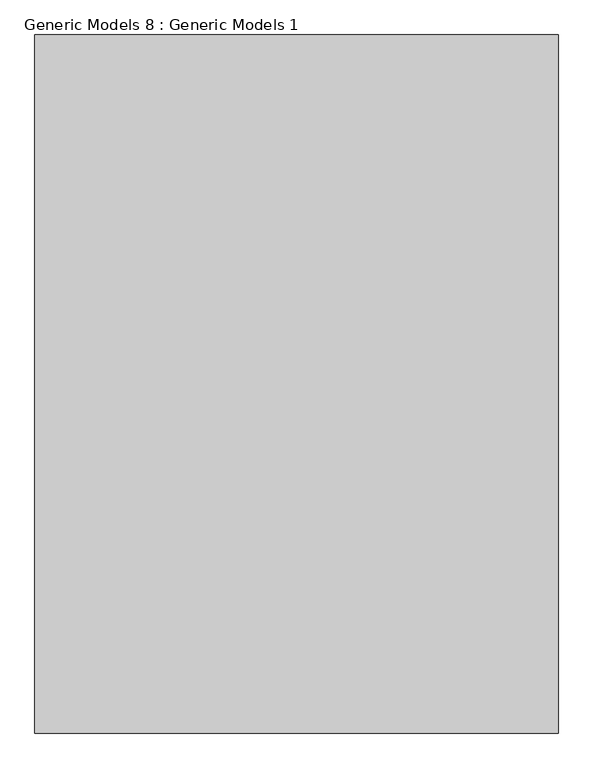
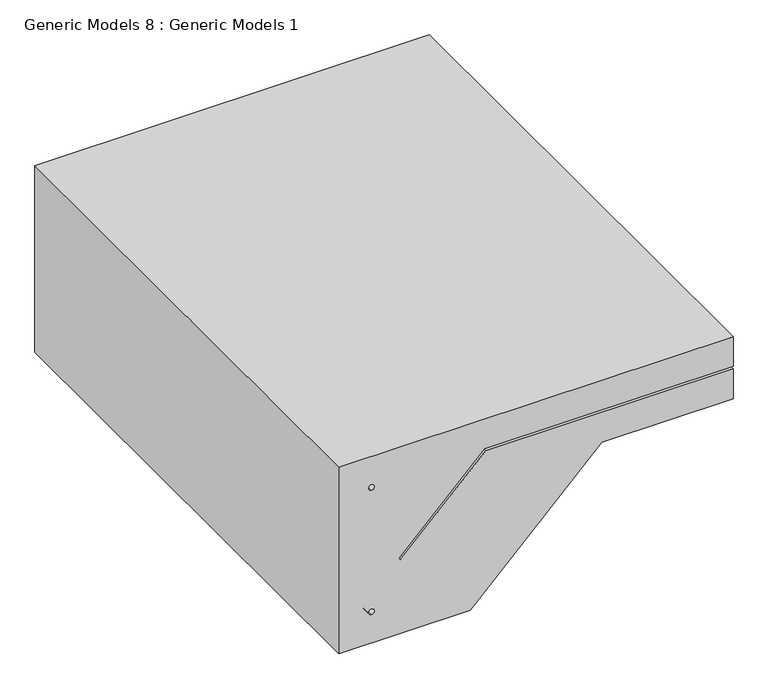
"""IFC4 building model written with IfcOpenShell, lengths in millimetres: proxy geometry, Generic Models 8 : Generic Models 1."""

import ifcopenshell
import ifcopenshell.guid

model = None  # the IFC model being written
_history = None  # IfcOwnerHistory: only IFC2X3 demands one
_inside = {}  # id of a spatial element -> (the spatial element, [elements in it])
_under = {}  # id of a project, library or spatial element -> (it, [spatial elements below it])
_declared = {}  # id of a project -> (the project, [libraries it declares])
_typed = {}  # id of a type object -> (the type object, [elements of that type])
_made_of = {}  # id of a material, layer set ... -> (it, [elements and type objects made of it])


def new_model(schema):
    """Start an empty IFC model of exactly this schema.

    Asked for "IFC4X3", IfcOpenShell would pick the latest addendum, in which some entities
    have other attributes; the version numbers below select the first issue.
    IFC2X3 requires an IfcOwnerHistory on every rooted entity: one is made here for all.
    """
    global model, _history
    if schema == "IFC4X3":
        model = ifcopenshell.file(schema_version=(4, 3, 0, 0))
    else:
        model = ifcopenshell.file(schema=schema)
    _inside.clear()
    _under.clear()
    _declared.clear()
    _typed.clear()
    _made_of.clear()
    _history = None
    if model.schema == "IFC2X3":
        org = make("IfcOrganization", Name="unknown")
        user = make(
            "IfcPersonAndOrganization",
            ThePerson=make("IfcPerson", FamilyName="unknown"),
            TheOrganization=org,
        )
        app = make(
            "IfcApplication",
            ApplicationDeveloper=org,
            Version="unknown",
            ApplicationFullName="unknown",
            ApplicationIdentifier="unknown",
        )
        _history = make(
            "IfcOwnerHistory",
            OwningUser=user,
            OwningApplication=app,
            ChangeAction="ADDED",
            CreationDate=0,
        )
    return model


def make(cls, **values):
    """One entity of the class cls with the attributes given. An attribute that is None is left unset."""
    return model.create_entity(
        cls, **{name: value for name, value in values.items() if value is not None}
    )


def rooted(cls, **values):
    """An entity with a GlobalId (a new one), such as an element, a storey or a relation."""
    return make(cls, GlobalId=ifcopenshell.guid.new(), OwnerHistory=_history, **values)


def si_unit(unit_type, name, prefix=None):
    """IfcSIUnit, for example si_unit("LENGTHUNIT", "METRE", prefix="MILLI")."""
    return make("IfcSIUnit", UnitType=unit_type, Prefix=prefix, Name=name)


def assignment(units):
    """IfcUnitAssignment: the units of a project."""
    return None if units is None else make("IfcUnitAssignment", Units=units)


def point(xyz):
    """IfcCartesianPoint."""
    return None if xyz is None else make("IfcCartesianPoint", Coordinates=xyz)


def direction(xyz):
    """IfcDirection."""
    return None if xyz is None else make("IfcDirection", DirectionRatios=xyz)


def frame(location, z_axis=None, x_axis=None):
    """IfcAxis2Placement3D, a coordinate frame: its origin and axes. An axis left out is left unset."""
    return make(
        "IfcAxis2Placement3D",
        Location=point(location),
        Axis=direction(z_axis),
        RefDirection=direction(x_axis),
    )


def frame_2d(location, x_axis=None):
    """IfcAxis2Placement2D, a coordinate frame in the plane: its origin and x axis."""
    return make(
        "IfcAxis2Placement2D", Location=point(location), RefDirection=direction(x_axis)
    )


def origin():
    """The frame at (0, 0, 0) with its axes left unset."""
    return frame((0.0, 0.0, 0.0))


def place(relative_to, where):
    """IfcLocalPlacement: puts the frame where relative to a parent placement (None: the world)."""
    return make(
        "IfcLocalPlacement", PlacementRelTo=relative_to, RelativePlacement=where
    )


def context(
    kind, dimensions, precision=None, world=None, true_north=None, identifier=None
):
    """IfcGeometricRepresentationContext, for example the 3D "Model" context."""
    return make(
        "IfcGeometricRepresentationContext",
        ContextIdentifier=identifier,
        ContextType=kind,
        CoordinateSpaceDimension=dimensions,
        Precision=precision,
        WorldCoordinateSystem=world,
        TrueNorth=true_north,
    )


def project(units=None, contexts=None):
    """IfcProject with its units and contexts."""
    return rooted(
        "IfcProject",
        Name="project",
        RepresentationContexts=contexts,
        UnitsInContext=assignment(units),
    )


def spatial(cls, under=None, at=None, **own):
    """A site, building, storey or space (cls), placed at a placement, below another one or the project."""
    s = rooted(cls, ObjectPlacement=at, **own)
    if under is not None:
        _under.setdefault(under.id(), (under, []))[1].append(s)
    return s


def polyline(points):
    """IfcPolyline through the points."""
    return make("IfcPolyline", Points=[point(p) for p in points])


def circle_curve(where, radius):
    """IfcCircle in the frame where."""
    return make("IfcCircle", Position=where, Radius=radius)


def trimmed(basis, trim1, trim2, sense, master):
    """IfcTrimmedCurve: the piece of a basis curve between two trims."""
    return make(
        "IfcTrimmedCurve",
        BasisCurve=basis,
        Trim1=trim1,
        Trim2=trim2,
        SenseAgreement=sense,
        MasterRepresentation=master,
    )


def segment(curve, same_sense, transition):
    """IfcCompositeCurveSegment."""
    return make(
        "IfcCompositeCurveSegment",
        Transition=transition,
        SameSense=same_sense,
        ParentCurve=curve,
    )


def composite_curve(segments, self_intersect=None):
    """IfcCompositeCurve: segments joined end to end."""
    return make("IfcCompositeCurve", Segments=segments, SelfIntersect=self_intersect)


def outline(outer, holes=None, kind="AREA"):
    """IfcArbitraryClosedProfileDef: a profile drawn as a closed curve; with holes, ...WithVoids."""
    if holes is None:
        return make("IfcArbitraryClosedProfileDef", ProfileType=kind, OuterCurve=outer)
    return make(
        "IfcArbitraryProfileDefWithVoids",
        ProfileType=kind,
        OuterCurve=outer,
        InnerCurves=holes,
    )


def extrude(swept, where, along, depth):
    """IfcExtrudedAreaSolid: the profile swept, set in the frame where, extruded along a direction by depth."""
    return make(
        "IfcExtrudedAreaSolid",
        SweptArea=swept,
        Position=where,
        ExtrudedDirection=direction(along),
        Depth=depth,
    )


def shape(context_of_items, identifier, shape_type, items):
    """IfcShapeRepresentation: the items that make up one representation, for example the "Body"."""
    return make(
        "IfcShapeRepresentation",
        ContextOfItems=context_of_items,
        RepresentationIdentifier=identifier,
        RepresentationType=shape_type,
        Items=items,
    )


def source(mapping_origin, context_of_items, identifier, shape_type, items):
    """IfcRepresentationMap: a shape defined once, which mapped items show again and again."""
    return make(
        "IfcRepresentationMap",
        MappingOrigin=mapping_origin,
        MappedRepresentation=shape(context_of_items, identifier, shape_type, items),
    )


def transform(
    local_origin,
    x_axis=None,
    y_axis=None,
    z_axis=None,
    scale=None,
    scale2=None,
    scale3=None,
    uniform=True,
):
    """IfcCartesianTransformationOperator3D, or its non-uniform kind. x_axis, y_axis, z_axis: its Axis1, 2, 3."""
    if uniform:
        return make(
            "IfcCartesianTransformationOperator3D",
            Axis1=direction(x_axis),
            Axis2=direction(y_axis),
            LocalOrigin=point(local_origin),
            Scale=scale,
            Axis3=direction(z_axis),
        )
    return make(
        "IfcCartesianTransformationOperator3DnonUniform",
        Axis1=direction(x_axis),
        Axis2=direction(y_axis),
        LocalOrigin=point(local_origin),
        Scale=scale,
        Axis3=direction(z_axis),
        Scale2=scale2,
        Scale3=scale3,
    )


def mapped(mapping_source, mapping_target):
    """IfcMappedItem: shows the shape of a source again, moved by a transform."""
    return make(
        "IfcMappedItem", MappingSource=mapping_source, MappingTarget=mapping_target
    )


def made_of(thing, what):
    """Note that an element or type object is made of a material, layer set ...; save() writes the relation."""
    if what is not None:
        _made_of.setdefault(what.id(), (what, []))[1].append(thing)
    return thing


def element(
    cls,
    number,
    at=None,
    inside=None,
    cuts=None,
    type_object=None,
    material=None,
    context=None,
    identifier="Body",
    shape_type=None,
    held_by="IfcProductDefinitionShape",
    body=None,
    shapes=None,
    **own,
):
    """One element of the class cls, such as IfcWall. Its Tag is "e" and its number.

    at: its placement. inside: the storey or other place that contains it. cuts: it is an
    opening in that element (IfcRelVoidsElement). A single representation is given by context,
    identifier, shape_type and body (its items); several are given by shapes. held_by: the class
    of the entity that holds the representations. save() writes the other relations.
    """
    e = rooted(cls, Tag="e%d" % number, ObjectPlacement=at, **own)
    if body is not None:
        shapes = [shape(context, identifier, shape_type, body)]
    if shapes is not None:
        e.Representation = make(held_by, Representations=shapes)
    if inside is not None:
        _inside.setdefault(inside.id(), (inside, []))[1].append(e)
    if cuts is not None:
        rooted(
            "IfcRelVoidsElement", RelatingBuildingElement=cuts, RelatedOpeningElement=e
        )
    if type_object is not None:
        _typed.setdefault(type_object.id(), (type_object, []))[1].append(e)
    return made_of(e, material)


def aggregate(whole, parts):
    """IfcRelAggregates: a whole, such as a stair, and the parts it consists of."""
    return rooted("IfcRelAggregates", RelatingObject=whole, RelatedObjects=parts)


def save(model, path):
    """Write the relations noted so far, then the file.

    IfcRelAggregates (storeys below a building ...), IfcRelContainedInSpatialStructure (elements
    in a storey), IfcRelDefinesByType, IfcRelAssociatesMaterial and IfcRelDeclares: one each for
    every whole, place, type object, material and project.
    """
    for whole, parts in _under.values():
        aggregate(whole, parts)
    for where, things in _inside.values():
        rooted(
            "IfcRelContainedInSpatialStructure",
            RelatedElements=things,
            RelatingStructure=where,
        )
    for kind, things in _typed.values():
        rooted("IfcRelDefinesByType", RelatedObjects=things, RelatingType=kind)
    for what, things in _made_of.values():
        rooted("IfcRelAssociatesMaterial", RelatedObjects=things, RelatingMaterial=what)
    for by, libraries in _declared.values():
        rooted("IfcRelDeclares", RelatingContext=by, RelatedDefinitions=libraries)
    model.write(path)


def generic_models_8_generic_models_1_dd7fddfd(model_context):
    return source(origin(), model_context, "Body", "SweptSolid", [
        extrude(outline(polyline([(0.0, 52785.9625), (0.0, 51871.5625), (-457.2, 51871.5625), (-457.2, 52176.3625), (-152.4, 52481.1625), (-152.4, 52785.9625), (-79.375, 52785.9625), (-79.375, 52212.2583259), (-276.674432, 52014.9588939), (-272.1843039, 52010.4687659), (-73.025, 52209.6280698), (-73.025, 52785.9625), (0.0, 52785.9625)]), holes=[composite_curve([segment(trimmed(circle_curve(frame_2d((-76.2, 51947.7625)), 6.35), [point((-69.85, 51947.7625))], [point((-82.55, 51947.7625))], True, "CARTESIAN"), True, "CONTINUOUS"), segment(trimmed(circle_curve(frame_2d((-76.2, 51947.7625)), 6.35), [point((-82.55, 51947.7625))], [point((-69.85, 51947.7625))], True, "CARTESIAN"), True, "CONTINUOUS")], self_intersect=False), composite_curve([segment(trimmed(circle_curve(frame_2d((-381.0, 51947.7625)), 6.35), [point((-374.65, 51947.7625))], [point((-387.35, 51947.7625))], True, "CARTESIAN"), True, "CONTINUOUS"), segment(trimmed(circle_curve(frame_2d((-381.0, 51947.7625)), 6.35), [point((-387.35, 51947.7625))], [point((-374.65, 51947.7625))], True, "CARTESIAN"), True, "CONTINUOUS")], self_intersect=False)]), frame((0.0, 0.0, 0.0), z_axis=(0.0, 1.0, 0.0), x_axis=(0.0, 0.0, 1.0)), (0.0, 0.0, 1.0), 1219.2),
    ])


if __name__ == "__main__":
    model = new_model("IFC4")
    model_context = context("Model", 3, world=origin())
    ifc_project = project(units=[si_unit("LENGTHUNIT", "METRE", prefix="MILLI")], contexts=[model_context])
    site = spatial("IfcSite", under=ifc_project)
    building = spatial("IfcBuilding", under=site)
    placement = place(None, origin())
    generic_models_8_generic_models_1_shape = generic_models_8_generic_models_1_dd7fddfd(model_context)
    element("IfcBuildingElementProxy", 1, Name="Generic Models 8 : Generic Models 1", ObjectType="Generic Models 8 : Generic Models 1", at=placement, inside=building, context=model_context, shape_type="MappedRepresentation", body=[
        mapped(generic_models_8_generic_models_1_shape, transform((0.0, 0.0, 0.0), x_axis=(1.0, 0.0, 0.0), y_axis=(0.0, 1.0, 0.0), z_axis=(0.0, 0.0, 1.0))),
    ])
    save(model, "model.ifc")

# Revit data of these elements
# Element 1 (IfcBuildingElementProxy, "Generic Models 8 : Generic Models 1")
#   Materials on its faces: "CONCRETE (3000 PSI CONCRETE)", "#10 6x6 WIRE MESH", "#4 CONT. STEEL REBAR"
# Materials
#   "CONCRETE (3000 PSI CONCRETE)": class "Concrete", colour RGB 192 192 192, transparency 0, Description = "Cast-in-place concrete", Cost = 0
#   "#10 6x6 WIRE MESH": class "Metal", colour RGB 189 187 185, transparency 0, Description = "Structural steel 50ksi", Cost = 0
#   "#4 CONT. STEEL REBAR": class "Metal", colour RGB 189 187 185, transparency 0, Description = "Structural steel 50ksi", Cost = 0
